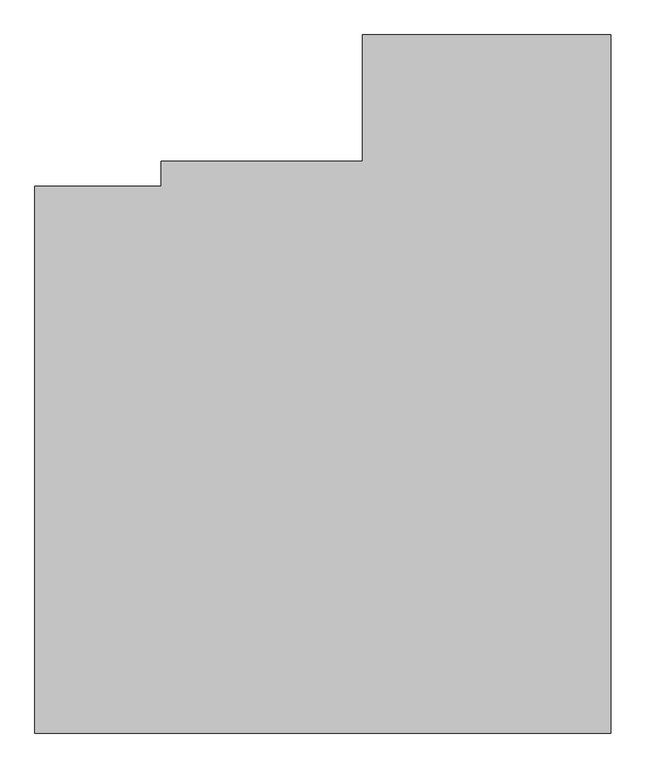
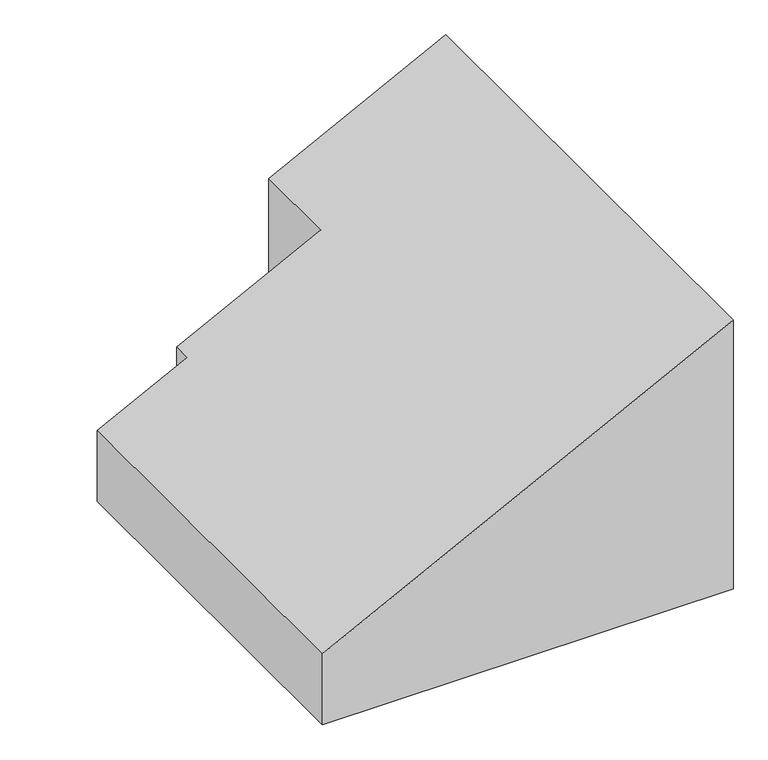
"""IFC4 building model written with IfcOpenShell, lengths in millimetres: proxy geometry, 0_3d_modell."""

import ifcopenshell
import ifcopenshell.guid

model = None  # the IFC model being written
_history = None  # IfcOwnerHistory: only IFC2X3 demands one
_inside = {}  # id of a spatial element -> (the spatial element, [elements in it])
_under = {}  # id of a project, library or spatial element -> (it, [spatial elements below it])
_declared = {}  # id of a project -> (the project, [libraries it declares])
_typed = {}  # id of a type object -> (the type object, [elements of that type])
_made_of = {}  # id of a material, layer set ... -> (it, [elements and type objects made of it])


def new_model(schema):
    """Start an empty IFC model of exactly this schema.

    Asked for "IFC4X3", IfcOpenShell would pick the latest addendum, in which some entities
    have other attributes; the version numbers below select the first issue.
    IFC2X3 requires an IfcOwnerHistory on every rooted entity: one is made here for all.
    """
    global model, _history
    if schema == "IFC4X3":
        model = ifcopenshell.file(schema_version=(4, 3, 0, 0))
    else:
        model = ifcopenshell.file(schema=schema)
    _inside.clear()
    _under.clear()
    _declared.clear()
    _typed.clear()
    _made_of.clear()
    _history = None
    if model.schema == "IFC2X3":
        org = make("IfcOrganization", Name="unknown")
        user = make(
            "IfcPersonAndOrganization",
            ThePerson=make("IfcPerson", FamilyName="unknown"),
            TheOrganization=org,
        )
        app = make(
            "IfcApplication",
            ApplicationDeveloper=org,
            Version="unknown",
            ApplicationFullName="unknown",
            ApplicationIdentifier="unknown",
        )
        _history = make(
            "IfcOwnerHistory",
            OwningUser=user,
            OwningApplication=app,
            ChangeAction="ADDED",
            CreationDate=0,
        )
    return model


def make(cls, **values):
    """One entity of the class cls with the attributes given. An attribute that is None is left unset."""
    return model.create_entity(
        cls, **{name: value for name, value in values.items() if value is not None}
    )


def rooted(cls, **values):
    """An entity with a GlobalId (a new one), such as an element, a storey or a relation."""
    return make(cls, GlobalId=ifcopenshell.guid.new(), OwnerHistory=_history, **values)


def si_unit(unit_type, name, prefix=None):
    """IfcSIUnit, for example si_unit("LENGTHUNIT", "METRE", prefix="MILLI")."""
    return make("IfcSIUnit", UnitType=unit_type, Prefix=prefix, Name=name)


def assignment(units):
    """IfcUnitAssignment: the units of a project."""
    return None if units is None else make("IfcUnitAssignment", Units=units)


def point(xyz):
    """IfcCartesianPoint."""
    return None if xyz is None else make("IfcCartesianPoint", Coordinates=xyz)


def direction(xyz):
    """IfcDirection."""
    return None if xyz is None else make("IfcDirection", DirectionRatios=xyz)


def frame(location, z_axis=None, x_axis=None):
    """IfcAxis2Placement3D, a coordinate frame: its origin and axes. An axis left out is left unset."""
    return make(
        "IfcAxis2Placement3D",
        Location=point(location),
        Axis=direction(z_axis),
        RefDirection=direction(x_axis),
    )


def origin():
    """The frame at (0, 0, 0) with its axes left unset."""
    return frame((0.0, 0.0, 0.0))


def place(relative_to, where):
    """IfcLocalPlacement: puts the frame where relative to a parent placement (None: the world)."""
    return make(
        "IfcLocalPlacement", PlacementRelTo=relative_to, RelativePlacement=where
    )


def context(
    kind, dimensions, precision=None, world=None, true_north=None, identifier=None
):
    """IfcGeometricRepresentationContext, for example the 3D "Model" context."""
    return make(
        "IfcGeometricRepresentationContext",
        ContextIdentifier=identifier,
        ContextType=kind,
        CoordinateSpaceDimension=dimensions,
        Precision=precision,
        WorldCoordinateSystem=world,
        TrueNorth=true_north,
    )


def project(units=None, contexts=None):
    """IfcProject with its units and contexts."""
    return rooted(
        "IfcProject",
        Name="project",
        RepresentationContexts=contexts,
        UnitsInContext=assignment(units),
    )


def spatial(cls, under=None, at=None, **own):
    """A site, building, storey or space (cls), placed at a placement, below another one or the project."""
    s = rooted(cls, ObjectPlacement=at, **own)
    if under is not None:
        _under.setdefault(under.id(), (under, []))[1].append(s)
    return s


def faces_of(points, faces, orient=None, outer=None):
    """IfcFace entities. A face is a list of loops; a loop is a list of indices into points, from 0.

    orient and outer hold one flag for each loop. By default every Orientation is true, the
    first loop of a face is its IfcFaceOuterBound and the others are IfcFaceBound.
    """
    made = []
    for i, loops in enumerate(faces):
        bounds = []
        for j, loop in enumerate(loops):
            is_outer = j == 0 if outer is None else outer[i][j]
            bounds.append(
                make(
                    "IfcFaceOuterBound" if is_outer else "IfcFaceBound",
                    Bound=make("IfcPolyLoop", Polygon=[points[k] for k in loop]),
                    Orientation=True if orient is None else orient[i][j],
                )
            )
        made.append(make("IfcFace", Bounds=bounds))
    return made


def faceted_brep(points, faces, orient=None, outer=None, voids=None):
    """IfcFacetedBrep: a solid bounded by flat faces; with voids (closed shells), ...WithVoids."""
    shared = [point(p) for p in points]
    hull = make("IfcClosedShell", CfsFaces=faces_of(shared, faces, orient, outer))
    if voids is None:
        return make("IfcFacetedBrep", Outer=hull)
    return make(
        "IfcFacetedBrepWithVoids",
        Outer=hull,
        Voids=[
            make(cls, CfsFaces=faces_of(shared, fs, o, b)) for cls, fs, o, b in voids
        ],
    )


def shape(context_of_items, identifier, shape_type, items):
    """IfcShapeRepresentation: the items that make up one representation, for example the "Body"."""
    return make(
        "IfcShapeRepresentation",
        ContextOfItems=context_of_items,
        RepresentationIdentifier=identifier,
        RepresentationType=shape_type,
        Items=items,
    )


def source(mapping_origin, context_of_items, identifier, shape_type, items):
    """IfcRepresentationMap: a shape defined once, which mapped items show again and again."""
    return make(
        "IfcRepresentationMap",
        MappingOrigin=mapping_origin,
        MappedRepresentation=shape(context_of_items, identifier, shape_type, items),
    )


def transform(
    local_origin,
    x_axis=None,
    y_axis=None,
    z_axis=None,
    scale=None,
    scale2=None,
    scale3=None,
    uniform=True,
):
    """IfcCartesianTransformationOperator3D, or its non-uniform kind. x_axis, y_axis, z_axis: its Axis1, 2, 3."""
    if uniform:
        return make(
            "IfcCartesianTransformationOperator3D",
            Axis1=direction(x_axis),
            Axis2=direction(y_axis),
            LocalOrigin=point(local_origin),
            Scale=scale,
            Axis3=direction(z_axis),
        )
    return make(
        "IfcCartesianTransformationOperator3DnonUniform",
        Axis1=direction(x_axis),
        Axis2=direction(y_axis),
        LocalOrigin=point(local_origin),
        Scale=scale,
        Axis3=direction(z_axis),
        Scale2=scale2,
        Scale3=scale3,
    )


def mapped(mapping_source, mapping_target):
    """IfcMappedItem: shows the shape of a source again, moved by a transform."""
    return make(
        "IfcMappedItem", MappingSource=mapping_source, MappingTarget=mapping_target
    )


def made_of(thing, what):
    """Note that an element or type object is made of a material, layer set ...; save() writes the relation."""
    if what is not None:
        _made_of.setdefault(what.id(), (what, []))[1].append(thing)
    return thing


def element(
    cls,
    number,
    at=None,
    inside=None,
    cuts=None,
    type_object=None,
    material=None,
    context=None,
    identifier="Body",
    shape_type=None,
    held_by="IfcProductDefinitionShape",
    body=None,
    shapes=None,
    **own,
):
    """One element of the class cls, such as IfcWall. Its Tag is "e" and its number.

    at: its placement. inside: the storey or other place that contains it. cuts: it is an
    opening in that element (IfcRelVoidsElement). A single representation is given by context,
    identifier, shape_type and body (its items); several are given by shapes. held_by: the class
    of the entity that holds the representations. save() writes the other relations.
    """
    e = rooted(cls, Tag="e%d" % number, ObjectPlacement=at, **own)
    if body is not None:
        shapes = [shape(context, identifier, shape_type, body)]
    if shapes is not None:
        e.Representation = make(held_by, Representations=shapes)
    if inside is not None:
        _inside.setdefault(inside.id(), (inside, []))[1].append(e)
    if cuts is not None:
        rooted(
            "IfcRelVoidsElement", RelatingBuildingElement=cuts, RelatedOpeningElement=e
        )
    if type_object is not None:
        _typed.setdefault(type_object.id(), (type_object, []))[1].append(e)
    return made_of(e, material)


def aggregate(whole, parts):
    """IfcRelAggregates: a whole, such as a stair, and the parts it consists of."""
    return rooted("IfcRelAggregates", RelatingObject=whole, RelatedObjects=parts)


def save(model, path):
    """Write the relations noted so far, then the file.

    IfcRelAggregates (storeys below a building ...), IfcRelContainedInSpatialStructure (elements
    in a storey), IfcRelDefinesByType, IfcRelAssociatesMaterial and IfcRelDeclares: one each for
    every whole, place, type object, material and project.
    """
    for whole, parts in _under.values():
        aggregate(whole, parts)
    for where, things in _inside.values():
        rooted(
            "IfcRelContainedInSpatialStructure",
            RelatedElements=things,
            RelatingStructure=where,
        )
    for kind, things in _typed.values():
        rooted("IfcRelDefinesByType", RelatedObjects=things, RelatingType=kind)
    for what, things in _made_of.values():
        rooted("IfcRelAssociatesMaterial", RelatedObjects=things, RelatingMaterial=what)
    for by, libraries in _declared.values():
        rooted("IfcRelDeclares", RelatingContext=by, RelatedDefinitions=libraries)
    model.write(path)


def generic_models_fb7019a2(model_context):
    return source(origin(), model_context, "Body", "Brep", [
        faceted_brep([(4680.0, 5670.0, 3237.913011), (2664.6018366, 5670.0, 2211.0163558), (2664.6018366, 4645.0, 2211.0163558), (1025.0, 4645.0, 1375.5974931), (1025.0, 4440.2642941, 1375.5974931), (0.0, 4440.2642941, 853.3339073), (0.0, 0.0, 853.3339073), (4680.0, 0.0, 3237.913011), (1025.0, 4440.2642941, 0.0), (0.0, 4440.2642941, 0.0), (1025.0, 4645.0, 0.0), (2664.6018366, 4645.0, 0.0), (2664.6018366, 5670.0, 0.0), (4680.0, 5670.0, 0.0), (4680.0, 0.0, 0.0), (0.0, 0.0, 0.0)], [[[0, 1, 2, 3, 4, 5, 6, 7]], [[5, 4, 8, 9]], [[4, 3, 10, 8]], [[3, 2, 11, 10]], [[2, 1, 12, 11]], [[1, 0, 13, 12]], [[14, 13, 0, 7]], [[7, 6, 15, 14]], [[6, 5, 9, 15]], [[11, 12, 13, 14, 15, 9, 8, 10]]]),
    ])


if __name__ == "__main__":
    model = new_model("IFC4")
    model_context = context("Model", 3, world=origin())
    ifc_project = project(units=[si_unit("LENGTHUNIT", "METRE", prefix="MILLI")], contexts=[model_context])
    site = spatial("IfcSite", under=ifc_project)
    building = spatial("IfcBuilding", under=site)
    placement = place(None, origin())
    generic_models_shape = generic_models_fb7019a2(model_context)
    element("IfcBuildingElementProxy", 1, Name="0_3d_modell", ObjectType="0_3d_modell", at=placement, inside=building, context=model_context, shape_type="MappedRepresentation", body=[
        mapped(generic_models_shape, transform((0.0, 0.0, 0.0), x_axis=(1.0, 0.0, 0.0), y_axis=(0.0, 1.0, 0.0), z_axis=(0.0, 0.0, 1.0))),
    ])
    save(model, "model.ifc")

# Revit data of these elements
# Element 1 (IfcBuildingElementProxy, "0_3d_modell")
#   Materials on its faces: "*1"
# Materials
#   "*1": class "Unassigned", colour RGB 175 175 175, transparency 0
